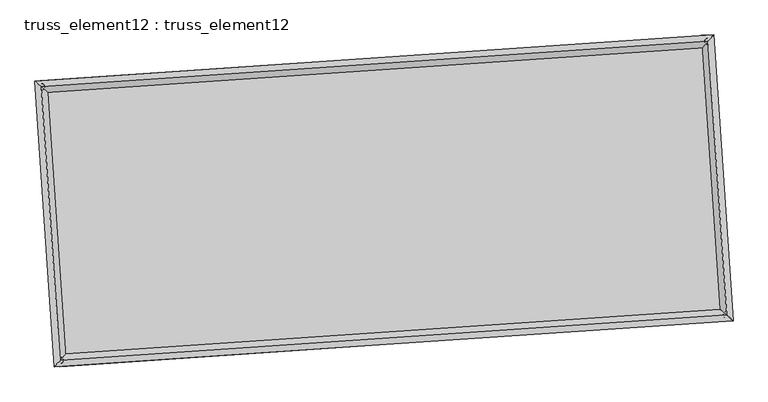
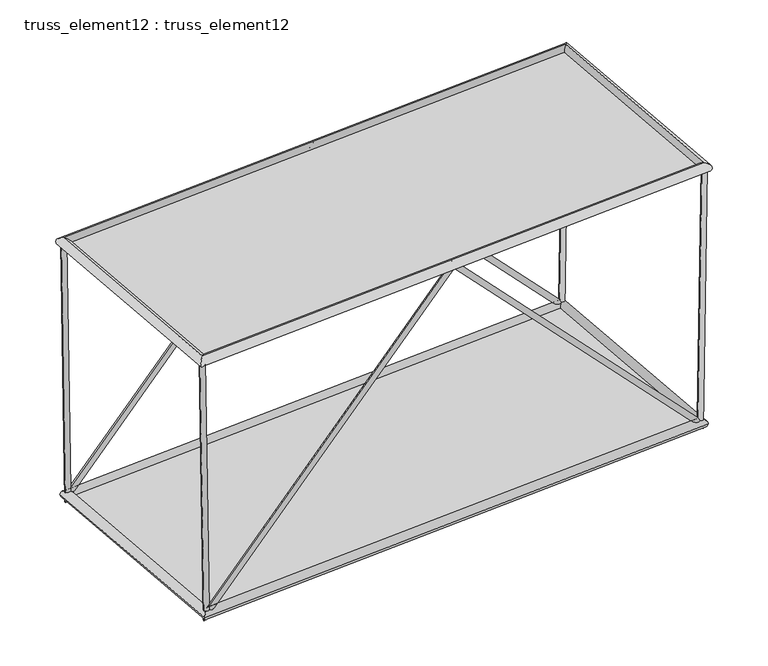
"""IFC4 building model written with IfcOpenShell, lengths in millimetres: plate geometry, truss_element12 : truss_element12."""

from ifc_helpers import new_model, si_unit, frame, origin, origin_with_axes, place, context, project, spatial, polyline, circle_curve, ellipse_curve, outline, extrude, source, transform, mapped, element, save
from ifc_brep_helpers import plane_surface, cylinder_surface, advanced_brep


def truss_element12_truss_element12_63e3ad5e(model_context):
    return source(origin(), model_context, "Body", "SolidModel", [
        advanced_brep(
        [(-3743.5185923, 2270.8661209, 5000.1655763), (-3842.6096052, 2257.5056903, 4998.5939367), (-3666.856189, 2276.0934388, 122.2062944), (-3762.1306939, 2262.9932413, -122.2062944), (1063.0344646, 2598.6067025, 5071.5097676), (1063.4928956, 2592.03417, 4927.2710279), (5794.2621458, 2921.211133, 122.2157479), (5890.4988312, 2921.1693555, -122.2157479), (5869.597537, 2926.3479669, 5000.17326), (5969.5853808, 2926.5619667, 4998.628818)],
        [
            (0, 1, circle_curve(frame((-3793.0640987, 2264.1859056, 4999.3797565), z_axis=(-0.01571413146651529, -0.0010714868896965779, 0.9998759513000092), x_axis=(-0.13360457302834886, 0.9910341776072246, -0.0010377284254098615)), 50.0)),
            (1, 0, circle_curve(frame((-3793.0640987, 2264.1859056, 4999.3797565), z_axis=(-0.01571413146651529, -0.0010714868896965779, 0.9998759513000092), x_axis=(-0.13360457302834886, 0.9910341776072246, -0.0010377284254098615)), 50.0)),
            (0, 2),
            (2, 3, ellipse_curve(frame((-3714.4934414, 2269.54334, 0.0), z_axis=(-0.9286913035150794, -0.06332392970054251, 0.3654073654193955), x_axis=(0.3645608612823961, 0.024858019305270502, 0.9308477089713743)), 131.5708228, 50.0)),
            (3, 1),
            (3, 2, ellipse_curve(frame((-3714.4934414, 2269.54334, 0.0), z_axis=(-0.9286913035150794, -0.06332392970054251, 0.3654073654193955), x_axis=(0.3645608612823961, 0.024858019305270502, 0.9308477089713743)), 131.5708228, 50.0)),
            (2, 4),
            (4, 5, ellipse_curve(frame((1063.2636801, 2595.3204362, 4999.3903977), z_axis=(-0.9976833935551674, -0.06802823805688821, -7.10712340997481e-05), x_axis=(7.090659019982544e-05, 4.834850845463915e-06, -0.9999999974744398)), 72.2764102, 50.0)),
            (5, 3),
            (5, 4, ellipse_curve(frame((1063.2636801, 2595.3204362, 4999.3903977), z_axis=(-0.9976833935551674, -0.06802823805688821, -7.10712340997481e-05), x_axis=(7.090659019982544e-05, 4.834850845463915e-06, -0.9999999974744398)), 72.2764102, 50.0)),
            (4, 6),
            (6, 7, ellipse_curve(frame((5842.3804885, 2921.1902443, 0.0), z_axis=(-0.928615683738225, -0.0633187734754156, -0.36560038955252466), x_axis=(-0.3647534382550607, -0.02487115039698468, 0.9307719136066805)), 131.5917158, 50.0)),
            (7, 5),
            (7, 6, ellipse_curve(frame((5842.3804885, 2921.1902443, 0.0), z_axis=(-0.928615683738225, -0.0633187734754156, -0.36560038955252466), x_axis=(-0.3647534382550607, -0.02487115039698468, 0.9307719136066805)), 131.5917158, 50.0)),
            (8, 9, circle_curve(frame((5919.5914589, 2926.4549668, 4999.401039), z_axis=(0.015442194086676379, 0.0010529445134941325, 0.999880207799735), x_axis=(-0.002156003891336237, 0.9999971558538857, -0.0010197702487463043)), 50.0)),
            (9, 8, circle_curve(frame((5919.5914589, 2926.4549668, 4999.401039), z_axis=(0.015442194086676379, 0.0010529445134941325, 0.999880207799735), x_axis=(-0.002156003891336237, 0.9999971558538857, -0.0010197702487463043)), 50.0)),
            (6, 8),
            (9, 7),
        ],
        [
            plane_surface(frame((-3793.0640987, 2314.1858769, 4999.4333375), z_axis=(-0.015714131466514486, -0.0010714868896970371, 0.9998759513000092), x_axis=(0.9998765254131398, -1.6839565107673603e-05, 0.015714122443711186))),
            cylinder_surface(frame((-3793.0640987, 2264.1859056, 4999.3797565), z_axis=(-0.015714131466515294, -0.001071486889696578, 0.9998759513000094), x_axis=(-0.13360457302834886, 0.9910341776072246, -0.0010377284254098615)), 50.0),
            cylinder_surface(frame((-3714.4934414, 2269.54334, 0.0), z_axis=(-0.6901348428855778, -0.047057671488220994, -0.7221492049357984), x_axis=(-0.02041190112427063, 0.9987523556187342, -0.04557506377968635)), 50.0),
            cylinder_surface(frame((1063.2636801, 2595.3204362, 4999.3903977), z_axis=(-0.6902372461888857, -0.04706465398020348, 0.7220508723901019), x_axis=(-0.11534249196066217, 0.9922793994945608, -0.04558182627998265)), 50.0),
            plane_surface(frame((5919.5914589, 2876.4549945, 4999.4536925), z_axis=(0.015442194086678164, 0.0010529445134923798, 0.9998802077997349), x_axis=(0.9998807622120697, -1.626171255075805e-05, -0.015442185524314327))),
            cylinder_surface(frame((5842.3804885, 2921.1902443, 0.0), z_axis=(-0.015442194086676379, -0.0010529445134941325, -0.999880207799735), x_axis=(-0.002156003891336237, 0.9999971558538857, -0.0010197702487463043)), 50.0),
        ],
        [
            (0, [[1, 2]]),
            (1, [[-1, 3, 4, 5]]),
            (1, [[-2, -5, 6, -3]]),
            (2, [[-4, 7, 8, 9]]),
            (2, [[-6, -9, 10, -7]]),
            (3, [[-8, 11, 12, 13]]),
            (3, [[-10, -13, 14, -11]]),
            (4, [[15, 16]]),
            (5, [[-12, 17, -16, 18]]),
            (5, [[-14, -18, -15, -17]]),
        ],
    ),
        advanced_brep(
        [(-3471.4056394, -1719.8674634, 5000.1655763), (-3570.4966523, -1733.227894, 4998.5939367), (-3394.7432361, -1714.6401455, 122.2062944), (-3490.0177409, -1727.740343, -122.2062944), (1335.1474175, -1392.1268818, 5071.5097676), (1335.6058485, -1398.6994143, 4927.2710279), (6066.3750987, -1069.5224513, 122.2157479), (6162.6117841, -1069.5642288, -122.2157479), (6141.71049, -1064.3856174, 5000.17326), (6241.6983337, -1064.1716176, 4998.628818)],
        [
            (0, 1, circle_curve(frame((-3520.9511458, -1726.5476787, 4999.3797565), z_axis=(-0.015714131466515315, -0.0010714868896965744, 0.9998759513000093), x_axis=(-0.1336045730283485, 0.9910341776072246, -0.0010377284254098622)), 50.0)),
            (1, 0, circle_curve(frame((-3520.9511458, -1726.5476787, 4999.3797565), z_axis=(-0.015714131466515315, -0.0010714868896965744, 0.9998759513000093), x_axis=(-0.1336045730283485, 0.9910341776072246, -0.0010377284254098622)), 50.0)),
            (0, 2),
            (2, 3, ellipse_curve(frame((-3442.3804885, -1721.1902443, 0.0), z_axis=(-0.9286913035150792, -0.06332392970054232, 0.3654073654193955), x_axis=(0.3645608612823961, 0.02485801930527043, 0.9308477089713744)), 131.5708228, 50.0)),
            (3, 1),
            (3, 2, ellipse_curve(frame((-3442.3804885, -1721.1902443, 0.0), z_axis=(-0.9286913035150792, -0.06332392970054232, 0.3654073654193955), x_axis=(0.3645608612823961, 0.02485801930527043, 0.9308477089713744)), 131.5708228, 50.0)),
            (2, 4),
            (4, 5, ellipse_curve(frame((1335.376633, -1395.4131481, 4999.3903977), z_axis=(-0.9976833935551673, -0.06802823805688811, -7.107123410030975e-05), x_axis=(7.090659020028672e-05, 4.8348508455792295e-06, -0.9999999974744398)), 72.2764102, 50.0)),
            (5, 3),
            (5, 4, ellipse_curve(frame((1335.376633, -1395.4131481, 4999.3903977), z_axis=(-0.9976833935551673, -0.06802823805688811, -7.107123410030975e-05), x_axis=(7.090659020028672e-05, 4.8348508455792295e-06, -0.9999999974744398)), 72.2764102, 50.0)),
            (4, 6),
            (6, 7, ellipse_curve(frame((6114.4934414, -1069.54334, 0.0), z_axis=(-0.9286156837382249, -0.06331877347541548, -0.36560038955252466), x_axis=(-0.3647534382550608, -0.024871150396984735, 0.9307719136066805)), 131.5917158, 50.0)),
            (7, 5),
            (7, 6, ellipse_curve(frame((6114.4934414, -1069.54334, 0.0), z_axis=(-0.9286156837382249, -0.06331877347541548, -0.36560038955252466), x_axis=(-0.3647534382550608, -0.024871150396984735, 0.9307719136066805)), 131.5917158, 50.0)),
            (8, 9, circle_curve(frame((6191.7044118, -1064.2786175, 4999.401039), z_axis=(0.015442194086677349, 0.001052944513494111, 0.999880207799735), x_axis=(-0.002156003891336467, 0.9999971558538856, -0.001019770248746277)), 50.0)),
            (9, 8, circle_curve(frame((6191.7044118, -1064.2786175, 4999.401039), z_axis=(0.015442194086677349, 0.001052944513494111, 0.999880207799735), x_axis=(-0.002156003891336467, 0.9999971558538856, -0.001019770248746277)), 50.0)),
            (6, 8),
            (9, 7),
        ],
        [
            plane_surface(frame((-3520.9511458, -1676.5477074, 4999.4333375), z_axis=(-0.015714131466514486, -0.001071486889697046, 0.9998759513000092), x_axis=(0.9998765254131398, -1.6839565107673603e-05, 0.015714122443711186))),
            cylinder_surface(frame((-3520.9511458, -1726.5476787, 4999.3797565), z_axis=(-0.015714131466515315, -0.0010714868896965744, 0.9998759513000093), x_axis=(-0.1336045730283485, 0.9910341776072246, -0.0010377284254098622)), 50.0),
            cylinder_surface(frame((-3442.3804885, -1721.1902443, 0.0), z_axis=(-0.6901348428855778, -0.04705767148822086, -0.7221492049357984), x_axis=(-0.020411901124270566, 0.9987523556187342, -0.045575063779686224)), 50.0),
            cylinder_surface(frame((1335.376633, -1395.4131481, 4999.3903977), z_axis=(-0.6902372461888866, -0.04706465398020354, 0.7220508723901011), x_axis=(-0.11534249196066206, 0.9922793994945608, -0.04558182627998265)), 50.0),
            plane_surface(frame((6191.7044118, -1114.2785898, 4999.4536925), z_axis=(0.015442194086678164, 0.0010529445134923896, 0.9998802077997349), x_axis=(0.9998807622120697, -1.6261712550313962e-05, -0.015442185524314327))),
            cylinder_surface(frame((6114.4934414, -1069.54334, 0.0), z_axis=(-0.015442194086677345, -0.0010529445134941108, -0.9998802077997347), x_axis=(-0.002156003891336467, 0.9999971558538856, -0.001019770248746277)), 50.0),
        ],
        [
            (0, [[1, 2]]),
            (1, [[-1, 3, 4, 5]]),
            (1, [[-2, -5, 6, -3]]),
            (2, [[-4, 7, 8, 9]]),
            (2, [[-6, -9, 10, -7]]),
            (3, [[-8, 11, 12, 13]]),
            (3, [[-10, -13, 14, -11]]),
            (4, [[15, 16]]),
            (5, [[-12, 17, -16, 18]]),
            (5, [[-14, -18, -15, -17]]),
        ],
    ),
        advanced_brep(
        [(-3520.9455782, -1726.5415079, 4909.3797567), (-3520.9567134, -1726.5538495, 5089.3797563), (-3793.0704524, 2264.1912635, 5089.3797563), (-3793.0577451, 2264.1805477, 4909.3797567), (5919.5966339, 2926.4611108, 5089.4010388), (5919.5862839, 2926.4488228, 4909.4010392), (6191.7103729, -1064.2840022, 5089.4010388), (6191.6984508, -1064.2732328, 4909.4010392)],
        [
            (0, 1, ellipse_curve(frame((-3520.9511458, -1726.5476787, 4999.3797565), z_axis=(-0.7535719234037697, 0.6573654662781985, -1.5458322817103875e-06), x_axis=(-0.6573654662763975, -0.7535719234053407, -1.5458322874531906e-06)), 127.2792206, 90.0)),
            (1, 2),
            (2, 3, ellipse_curve(frame((-3793.0640987, 2264.1859056, 4999.3797565), z_axis=(-0.6573654662763977, -0.7535719234053406, -1.5458322862734306e-06), x_axis=(0.7535719234037698, -0.6573654662781985, 1.5458322805306273e-06)), 127.2792206, 90.0)),
            (3, 0),
            (1, 0, ellipse_curve(frame((-3520.9511458, -1726.5476787, 4999.3797565), z_axis=(-0.7535719234037697, 0.6573654662781985, -1.5458322817103875e-06), x_axis=(-0.6573654662763975, -0.7535719234053407, -1.5458322874531906e-06)), 127.2792206, 90.0)),
            (3, 2, ellipse_curve(frame((-3793.0640987, 2264.1859056, 4999.3797565), z_axis=(-0.6573654662763977, -0.7535719234053406, -1.5458322862734306e-06), x_axis=(0.7535719234037698, -0.6573654662781985, 1.5458322805306273e-06)), 127.2792206, 90.0)),
            (2, 4),
            (4, 5, ellipse_curve(frame((5919.5914589, 2926.4549668, 4999.401039), z_axis=(-0.7535719234037713, 0.6573654662781966, -1.54583228340204e-06), x_axis=(-0.657365466276396, -0.7535719234053422, -1.5458322834020181e-06)), 127.2792206, 90.0)),
            (5, 3),
            (5, 4, ellipse_curve(frame((5919.5914589, 2926.4549668, 4999.401039), z_axis=(-0.7535719234037713, 0.6573654662781966, -1.54583228340204e-06), x_axis=(-0.657365466276396, -0.7535719234053422, -1.5458322834020181e-06)), 127.2792206, 90.0)),
            (4, 6),
            (6, 7, ellipse_curve(frame((6191.7044118, -1064.2786175, 4999.401039), z_axis=(0.657365466276396, 0.7535719234053422, 1.5458322845817783e-06), x_axis=(-0.7535719234037713, 0.6573654662781966, -1.5458322845818003e-06)), 127.2792206, 90.0)),
            (7, 5),
            (7, 6, ellipse_curve(frame((6191.7044118, -1064.2786175, 4999.401039), z_axis=(0.657365466276396, 0.7535719234053422, 1.5458322845817783e-06), x_axis=(-0.7535719234037713, 0.6573654662781966, -1.5458322845818003e-06)), 127.2792206, 90.0)),
            (6, 1),
            (0, 7),
        ],
        [
            cylinder_surface(frame((-3520.9511458, -1726.5476787, 4999.3797565), z_axis=(0.06802823822869807, -0.997683396074877, 0.0), x_axis=(-0.9976833938766201, -0.06802823807880728, -6.638314780363972e-05)), 90.0),
            cylinder_surface(frame((-3793.0640987, 2264.1859056, 4999.3797565), z_axis=(-0.9976833960724929, -0.06802823822853457, -2.1861369803413196e-06), x_axis=(-0.0680282379484979, 0.9976833940285698, -6.419701082374248e-05)), 90.0),
            cylinder_surface(frame((5919.5914589, 2926.4549668, 4999.401039), z_axis=(-0.06802823822870287, 0.9976833960748764, 0.0), x_axis=(0.9976833941566563, 0.06802823809790673, -6.201087384790602e-05)), 90.0),
            cylinder_surface(frame((6191.7044118, -1064.2786175, 4999.401039), z_axis=(0.9976833960724929, 0.06802823822853456, 2.1861369820097525e-06), x_axis=(0.06802823822853456, -0.9976833940094751, -6.4197010825411e-05)), 90.0),
        ],
        [
            (0, [[1, 2, 3, 4]]),
            (0, [[5, -4, 6, -2]]),
            (1, [[-3, 7, 8, 9]]),
            (1, [[-6, -9, 10, -7]]),
            (2, [[-8, 11, 12, 13]]),
            (2, [[-10, -13, 14, -11]]),
            (3, [[-12, 15, -1, 16]]),
            (3, [[-14, -16, -5, -15]]),
        ],
    ),
        advanced_brep(
        [(-3358.7115243, -1625.2761972, 0.0), (-3526.0494527, -1817.1042913, 0.0), (-3810.4074885, 2353.2123043, 0.0), (-3618.5793943, 2185.8743758, 0.0), (5926.0494527, 3017.1042913, 0.0), (5758.7115243, 2825.2761972, 0.0), (6210.4074885, -1153.2123043, 0.0), (6018.5793943, -985.8743758, 0.0)],
        [
            (0, 1, ellipse_curve(frame((-3442.3804885, -1721.1902443, 0.0), z_axis=(-0.7535719234054559, 0.6573654662780831, 0.0), x_axis=(-0.657365466278083, -0.7535719234054561, 0.0)), 127.2792206, 90.0)),
            (1, 2),
            (2, 3, ellipse_curve(frame((-3714.4934414, 2269.54334, 0.0), z_axis=(-0.657365466278083, -0.753571923405456, 0.0), x_axis=(0.753571923405456, -0.657365466278083, 0.0)), 127.2792206, 90.0)),
            (3, 0),
            (1, 0, ellipse_curve(frame((-3442.3804885, -1721.1902443, 0.0), z_axis=(-0.7535719234054559, 0.6573654662780831, 0.0), x_axis=(-0.657365466278083, -0.7535719234054561, 0.0)), 127.2792206, 90.0)),
            (3, 2, ellipse_curve(frame((-3714.4934414, 2269.54334, 0.0), z_axis=(-0.657365466278083, -0.753571923405456, 0.0), x_axis=(0.753571923405456, -0.657365466278083, 0.0)), 127.2792206, 90.0)),
            (2, 4),
            (4, 5, ellipse_curve(frame((5842.3804885, 2921.1902443, 0.0), z_axis=(-0.7535719234054572, 0.6573654662780815, 0.0), x_axis=(-0.6573654662780817, -0.7535719234054572, 0.0)), 127.2792206, 90.0)),
            (5, 3),
            (5, 4, ellipse_curve(frame((5842.3804885, 2921.1902443, 0.0), z_axis=(-0.7535719234054572, 0.6573654662780815, 0.0), x_axis=(-0.6573654662780817, -0.7535719234054572, 0.0)), 127.2792206, 90.0)),
            (4, 6),
            (6, 7, ellipse_curve(frame((6114.4934414, -1069.54334, 0.0), z_axis=(0.6573654662780816, 0.7535719234054572, 0.0), x_axis=(-0.7535719234054571, 0.6573654662780817, 0.0)), 127.2792206, 90.0)),
            (7, 5),
            (7, 6, ellipse_curve(frame((6114.4934414, -1069.54334, 0.0), z_axis=(0.6573654662780816, 0.7535719234054572, 0.0), x_axis=(-0.7535719234054571, 0.6573654662780817, 0.0)), 127.2792206, 90.0)),
            (6, 1),
            (0, 7),
        ],
        [
            cylinder_surface(frame((-3442.3804885, -1721.1902443, 0.0), z_axis=(0.06802823822869886, -0.9976833960748768, 0.0), x_axis=(-0.9976833960748768, -0.06802823822869886, 0.0)), 90.0),
            cylinder_surface(frame((-3714.4934414, 2269.54334, 0.0), z_axis=(-0.9976833960748769, -0.06802823822869761, 0.0), x_axis=(-0.06802823822869761, 0.9976833960748769, 0.0)), 90.0),
            cylinder_surface(frame((5842.3804885, 2921.1902443, 0.0), z_axis=(-0.06802823822870288, 0.9976833960748764, 0.0), x_axis=(0.9976833960748764, 0.06802823822870288, 0.0)), 90.0),
            cylinder_surface(frame((6114.4934414, -1069.54334, 0.0), z_axis=(0.9976833960748769, 0.06802823822869744, 0.0), x_axis=(0.06802823822869744, -0.9976833960748769, 0.0)), 90.0),
        ],
        [
            (0, [[1, 2, 3, 4]]),
            (0, [[5, -4, 6, -2]]),
            (1, [[-3, 7, 8, 9]]),
            (1, [[-6, -9, 10, -7]]),
            (2, [[-8, 11, 12, 13]]),
            (2, [[-10, -13, 14, -11]]),
            (3, [[-12, 15, -1, 16]]),
            (3, [[-14, -16, -5, -15]]),
        ],
    ),
        extrude(outline(polyline([(-3442.3804885, -1721.1902443), (-3714.4934414, 2269.54334), (5842.3804885, 2921.1902443), (6114.4934414, -1069.54334), (-3442.3804885, -1721.1902443)])), origin_with_axes(), (0.0, 0.0, 1.0), 20.0),
        extrude(outline(polyline([(-2000.0, 4867.6040896), (2000.0, 4867.6040896), (1999.9999999, -4867.6040895), (-2000.0000001, -4867.6040895), (-2000.0, 4867.6040896)])), frame((1199.3201566, 599.9536441, 4999.3903977), z_axis=(-2.1810725665555367e-06, -1.4871905135056997e-07, 0.9999999999976104), x_axis=(-0.0680282382286985, 0.9976833960748769, 0.0)), (0.0, 0.0, 1.0), 20.0),
    ])


if __name__ == "__main__":
    model = new_model("IFC4")
    model_context = context("Model", 3, world=origin())
    ifc_project = project(units=[si_unit("LENGTHUNIT", "METRE", prefix="MILLI")], contexts=[model_context])
    site = spatial("IfcSite", under=ifc_project)
    building = spatial("IfcBuilding", under=site)
    placement = place(None, origin())
    truss_element12_truss_element12_shape = truss_element12_truss_element12_63e3ad5e(model_context)
    element("IfcPlate", 1, ObjectType="truss_element12 : truss_element12", at=placement, inside=building, context=model_context, shape_type="MappedRepresentation", body=[
        mapped(truss_element12_truss_element12_shape, transform((0.0, 0.0, 0.0), x_axis=(1.0, 0.0, 0.0), y_axis=(0.0, 1.0, 0.0), z_axis=(0.0, 0.0, 1.0))),
    ])
    save(model, "model.ifc")

# Revit data of these elements
# Type "truss_element12 : truss_element12"
#   steellbar1 = 90 mm
#   steelbar2 = 50 mm
#   offset1 = 5000 mm
#   M = Default Roof
# Element 1 (IfcPlate, "truss_element12 : truss_element12")
#   Materials on its faces: "Default Roof"
# Materials
#   "Default Roof": class "Miscellaneous", colour RGB 0 127 0, transparency 0, Comments = "Rendering appearance not upgraded Rendering appearance not upgraded ", Cost = 0
